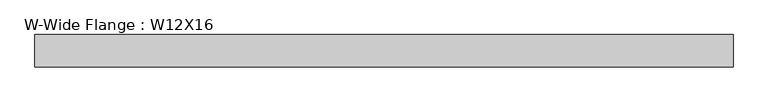
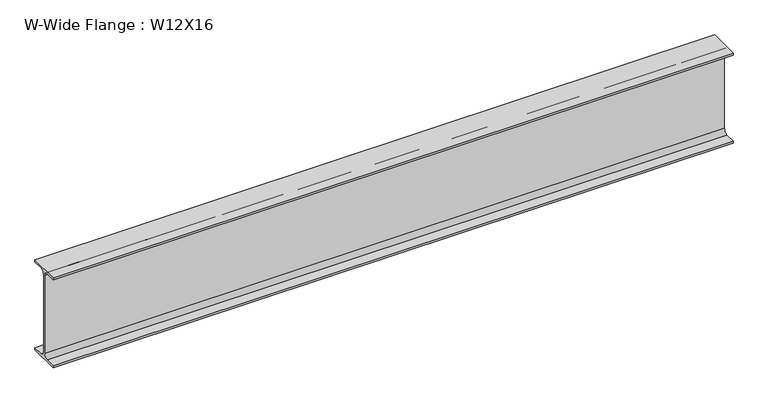
"""IFC4 building model written with IfcOpenShell, lengths in millimetres: beam geometry, W-Wide Flange : W12X16."""

from ifc_helpers import new_model, si_unit, point, frame, frame_2d, origin, place, context, project, spatial, polyline, circle_curve, trimmed, segment, composite_curve, outline, extrude, source, transform, mapped, element, save


def w_wide_flange_w12x16_59da3857(model_context):
    return source(origin(), model_context, "Body", "SweptSolid", [
        extrude(outline(composite_curve([segment(polyline([(50.673, -145.669), (50.673, -152.4), (-50.673, -152.4), (-50.673, -145.669), (-16.7005, -145.669)]), True, "CONTINUOUS"), segment(trimmed(circle_curve(frame_2d((-16.7005, -131.7625)), 13.9065), [point((-16.7005, -145.669))], [point((-2.794, -131.7625))], True, "CARTESIAN"), True, "CONTINUOUS"), segment(polyline([(-2.794, -131.7625), (-2.794, 131.7625)]), True, "CONTINUOUS"), segment(trimmed(circle_curve(frame_2d((-16.7005, 131.7625)), 13.9065), [point((-2.794, 131.7625))], [point((-16.7005, 145.669))], True, "CARTESIAN"), True, "CONTINUOUS"), segment(polyline([(-16.7005, 145.669), (-50.673, 145.669), (-50.673, 152.4), (50.673, 152.4), (50.673, 145.669), (16.7005, 145.669)]), True, "CONTINUOUS"), segment(trimmed(circle_curve(frame_2d((16.7005, 131.7625)), 13.9065), [point((16.7005, 145.669))], [point((2.794, 131.7625))], True, "CARTESIAN"), True, "CONTINUOUS"), segment(polyline([(2.794, 131.7625), (2.794, -131.7625)]), True, "CONTINUOUS"), segment(trimmed(circle_curve(frame_2d((16.7005, -131.7625)), 13.9065), [point((2.794, -131.7625))], [point((16.7005, -145.669))], True, "CARTESIAN"), True, "CONTINUOUS"), segment(polyline([(16.7005, -145.669), (50.673, -145.669)]), True, "CONTINUOUS")], self_intersect=False)), frame((-1062.7816406, 0.0, 0.0), z_axis=(1.0, 0.0, 0.0), x_axis=(0.0, 1.0, 0.0)), (0.0, 0.0, 1.0), 2175.5695313),
    ])


if __name__ == "__main__":
    model = new_model("IFC4")
    model_context = context("Model", 3, world=origin())
    ifc_project = project(units=[si_unit("LENGTHUNIT", "METRE", prefix="MILLI")], contexts=[model_context])
    site = spatial("IfcSite", under=ifc_project)
    building = spatial("IfcBuilding", under=site)
    placement = place(None, origin())
    w_wide_flange_w12x16_shape = w_wide_flange_w12x16_59da3857(model_context)
    element("IfcBeam", 1, ObjectType="W-Wide Flange : W12X16", at=placement, inside=building, context=model_context, shape_type="MappedRepresentation", body=[
        mapped(w_wide_flange_w12x16_shape, transform((0.0, 0.0, 0.0), x_axis=(1.0, 0.0, 0.0), y_axis=(0.0, 1.0, 0.0), z_axis=(0.0, 0.0, 1.0))),
    ])
    save(model, "model.ifc")

# Revit data of these elements
# Type "W-Wide Flange : W12X16"
#   Assembly Code = "B10"
#   W = 16
#   Length [instance default] = 1524 mm
#   bf = 101.346 mm
#   d = 304.8 mm
#   k = 20.638 mm
#   k2 = 13.907 mm
#   tf = 6.731 mm
#   tw = 5.588 mm
#   A = 0.0030387 m²
#   Structural Material [instance default] = Steel ASTM A992
# Element 1 (IfcBeam, "W-Wide Flange : W12X16")
#   Materials on its faces: "Steel ASTM A992"
# Materials
#   "Steel ASTM A992": class "Metal", colour RGB 128 0 0, transparency 0, Description = "Structural steel 50ksi", Cost = 0
